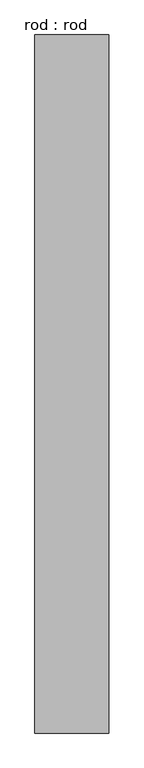
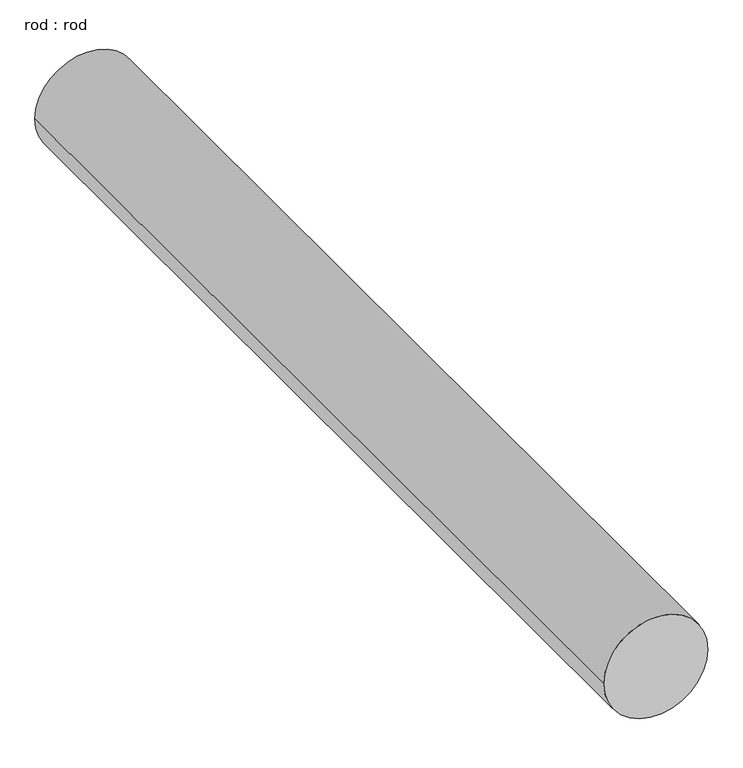
"""IFC4 building model written with IfcOpenShell, lengths in millimetres: proxy geometry, rod : rod."""

from ifc_helpers import new_model, si_unit, point, frame, frame_2d, origin, place, context, project, spatial, circle_curve, trimmed, segment, composite_curve, outline, extrude, source, transform, mapped, element, save


def rod_rod_045a65af(model_context):
    return source(origin(), model_context, "Body", "SweptSolid", [
        extrude(outline(composite_curve([segment(trimmed(circle_curve(frame_2d((0.0108462, 0.0)), 200.0), [point((0.0108462, 200.0))], [point((0.0108462, -200.0))], False, "CARTESIAN"), True, "CONTINUOUS"), segment(trimmed(circle_curve(frame_2d((0.0108462, 0.0)), 200.0), [point((0.0108462, -200.0))], [point((0.0108462, 200.0))], False, "CARTESIAN"), True, "CONTINUOUS")], self_intersect=False)), frame((0.0, 2204.3276845, 0.0), z_axis=(0.0, 1.0, 0.0), x_axis=(0.0, 0.0, 1.0)), (0.0, 0.0, 1.0), 3776.8018617),
    ])


if __name__ == "__main__":
    model = new_model("IFC4")
    model_context = context("Model", 3, world=origin())
    ifc_project = project(units=[si_unit("LENGTHUNIT", "METRE", prefix="MILLI")], contexts=[model_context])
    site = spatial("IfcSite", under=ifc_project)
    building = spatial("IfcBuilding", under=site)
    placement = place(None, origin())
    rod_rod_shape = rod_rod_045a65af(model_context)
    element("IfcBuildingElementProxy", 1, Name="rod : rod", ObjectType="rod : rod", at=placement, inside=building, context=model_context, shape_type="MappedRepresentation", body=[
        mapped(rod_rod_shape, transform((0.0, 0.0, 0.0), x_axis=(1.0, 0.0, 0.0), y_axis=(0.0, 1.0, 0.0), z_axis=(0.0, 0.0, 1.0))),
    ])
    save(model, "model.ifc")

# Revit data of these elements
# Type "rod : rod"
#   Default Elevation = 0
